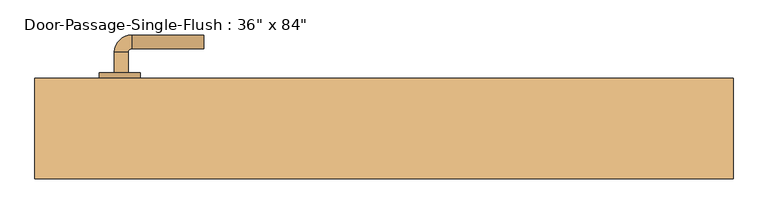
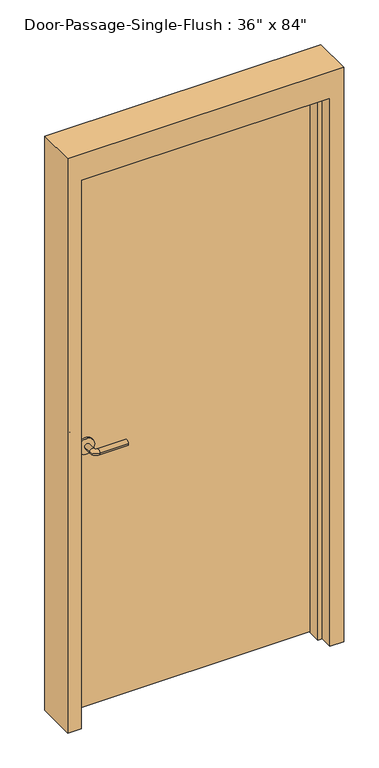
"""IFC4 building model written with IfcOpenShell, lengths in millimetres: door geometry."""

from ifc_helpers import new_model, si_unit, point, frame, frame_2d, origin, origin_with_axes, place, context, project, spatial, polyline, circle_curve, ellipse_curve, trimmed, segment, composite_curve, outline, extrude, faceted_brep, source, transform, mapped, element, save
from ifc_brep_helpers import plane_surface, cylinder_surface, revolved_surface, advanced_brep


def door_a856c21e(model_context):
    return source(origin(), model_context, "Body", "SolidModel", [
        advanced_brep(
        [(-392.190625, 80.9, 1016.0), (-372.190625, 80.9, 1016.0), (-372.190625, 50.9, 1016.0), (-392.190625, 50.9, 1016.0), (-367.190625, 45.9, 1016.0), (-367.190625, 25.9, 1016.0), (-262.190625, 25.9, 1016.0), (-262.190625, 45.9, 1016.0)],
        [
            (0, 1, circle_curve(frame((-382.190625, 80.9, 1016.0), z_axis=(0.0, 1.0, 0.0), x_axis=(1.0, 0.0, 0.0)), 10.0)),
            (1, 0, circle_curve(frame((-382.190625, 80.9, 1016.0), z_axis=(0.0, 1.0, 0.0), x_axis=(1.0, 0.0, 0.0)), 10.0)),
            (1, 2),
            (2, 3, circle_curve(frame((-382.190625, 50.9, 1016.0), z_axis=(0.0, 1.0, 0.0), x_axis=(1.0, 0.0, 0.0)), 10.0)),
            (3, 0),
            (3, 2, circle_curve(frame((-382.190625, 50.9, 1016.0), z_axis=(0.0, 1.0, 0.0), x_axis=(1.0, 0.0, 0.0)), 10.0)),
            (4, 5, circle_curve(frame((-367.190625, 35.9, 1016.0), z_axis=(-1.0, 0.0, 0.0), x_axis=(0.0, 1.0, 0.0)), 10.0)),
            (5, 3, circle_curve(frame((-367.190625, 50.9, 1016.0), z_axis=(0.0, 0.0, -1.0), x_axis=(-1.0, 0.0, 0.0)), 25.0)),
            (2, 4, circle_curve(frame((-367.190625, 50.9, 1016.0), z_axis=(0.0, 0.0, 1.0), x_axis=(-1.0, 0.0, 0.0)), 5.0)),
            (5, 4, circle_curve(frame((-367.190625, 35.9, 1016.0), z_axis=(-1.0, 0.0, 0.0), x_axis=(0.0, 1.0, 0.0)), 10.0)),
            (6, 7, circle_curve(frame((-262.190625, 35.9, 1016.0), z_axis=(1.0, 0.0, 0.0), x_axis=(0.0, 1.0, 0.0)), 10.0)),
            (7, 6, circle_curve(frame((-262.190625, 35.9, 1016.0), z_axis=(1.0, 0.0, 0.0), x_axis=(0.0, 1.0, 0.0)), 10.0)),
            (4, 7),
            (6, 5),
        ],
        [
            plane_surface(frame((-382.190625, 80.9, 1016.0), z_axis=(0.0, 1.0, 0.0), x_axis=(0.0, 0.0, 1.0))),
            cylinder_surface(frame((-382.190625, 80.9, 1016.0), z_axis=(0.0, 1.0, 0.0), x_axis=(1.0, 0.0, 0.0)), 10.0),
            revolved_surface(trimmed(ellipse_curve(frame((-382.190625, 50.9, 1016.0), z_axis=(0.0, -1.0, 0.0), x_axis=(1.0, 0.0, 0.0)), 10.0, 10.0), [point((-392.190625, 50.9, 1016.0))], [point((-372.190625, 50.9, 1016.0))], True, "CARTESIAN"), (-367.190625, 50.9, 1016.0), (0.0, 0.0, -1.0)),
            revolved_surface(trimmed(ellipse_curve(frame((-382.190625, 50.9, 1016.0), z_axis=(0.0, -1.0, 0.0), x_axis=(1.0, 0.0, 0.0)), 10.0, 10.0), [point((-372.190625, 50.9, 1016.0))], [point((-392.190625, 50.9, 1016.0))], True, "CARTESIAN"), (-367.190625, 50.9, 1016.0), (0.0, 0.0, -1.0)),
            plane_surface(frame((-262.190625, 35.9, 1016.0), z_axis=(1.0, 0.0, 0.0), x_axis=(0.0, 0.0, 1.0))),
            cylinder_surface(frame((-367.190625, 35.9, 1016.0), z_axis=(-1.0, 0.0, 0.0), x_axis=(0.0, 1.0, 0.0)), 10.0),
        ],
        [
            (0, [[1, 2]]),
            (1, [[3, 4, 5, -2]]),
            (1, [[-5, 6, -3, -1]]),
            (2, [[7, 8, -4, 9]]),
            (3, [[10, -9, -6, -8]]),
            (4, [[11, 12]]),
            (5, [[13, -11, 14, -7]]),
            (5, [[-14, -12, -13, -10]]),
        ],
    ),
        extrude(outline(composite_curve([segment(trimmed(circle_curve(frame_2d((1016.0, -384.690625)), 30.0), [point((1016.0, -414.690625))], [point((1016.0, -354.690625))], False, "CARTESIAN"), True, "CONTINUOUS"), segment(trimmed(circle_curve(frame_2d((1016.0, -384.690625)), 30.0), [point((1016.0, -354.690625))], [point((1016.0, -414.690625))], False, "CARTESIAN"), True, "CONTINUOUS")], self_intersect=False)), frame((0.0, 80.9, 0.0), z_axis=(0.0, 1.0, 0.0), x_axis=(0.0, 0.0, 1.0)), (0.0, 0.0, 1.0), 8.0),
        advanced_brep(
        [(-392.190625, 141.35, 1016.0), (-372.190625, 141.35, 1016.0), (-392.190625, 171.35, 1016.0), (-372.190625, 171.35, 1016.0), (-367.190625, 176.35, 1016.0), (-367.190625, 196.35, 1016.0), (-262.190625, 196.35, 1016.0), (-262.190625, 176.35, 1016.0)],
        [
            (0, 1, circle_curve(frame((-382.190625, 141.35, 1016.0), z_axis=(0.0, -1.0, 0.0), x_axis=(1.0, 0.0, 0.0)), 10.0)),
            (1, 0, circle_curve(frame((-382.190625, 141.35, 1016.0), z_axis=(0.0, -1.0, 0.0), x_axis=(1.0, 0.0, 0.0)), 10.0)),
            (0, 2),
            (2, 3, circle_curve(frame((-382.190625, 171.35, 1016.0), z_axis=(0.0, -1.0, 0.0), x_axis=(1.0, 0.0, 0.0)), 10.0)),
            (3, 1),
            (3, 2, circle_curve(frame((-382.190625, 171.35, 1016.0), z_axis=(0.0, -1.0, 0.0), x_axis=(1.0, 0.0, 0.0)), 10.0)),
            (4, 3, circle_curve(frame((-367.190625, 171.35, 1016.0), z_axis=(0.0, 0.0, 1.0), x_axis=(-1.0, 0.0, 0.0)), 5.0)),
            (2, 5, circle_curve(frame((-367.190625, 171.35, 1016.0), z_axis=(0.0, 0.0, -1.0), x_axis=(-1.0, 0.0, 0.0)), 25.0)),
            (5, 4, circle_curve(frame((-367.190625, 186.35, 1016.0), z_axis=(-1.0, 0.0, 0.0), x_axis=(0.0, -1.0, 0.0)), 10.0)),
            (4, 5, circle_curve(frame((-367.190625, 186.35, 1016.0), z_axis=(-1.0, 0.0, 0.0), x_axis=(0.0, -1.0, 0.0)), 10.0)),
            (6, 7, circle_curve(frame((-262.190625, 186.35, 1016.0), z_axis=(1.0, 0.0, 0.0), x_axis=(0.0, -1.0, 0.0)), 10.0)),
            (7, 6, circle_curve(frame((-262.190625, 186.35, 1016.0), z_axis=(1.0, 0.0, 0.0), x_axis=(0.0, -1.0, 0.0)), 10.0)),
            (5, 6),
            (7, 4),
        ],
        [
            plane_surface(frame((-382.190625, 141.35, 1016.0), z_axis=(0.0, -1.0, 0.0), x_axis=(0.0, 0.0, 1.0))),
            cylinder_surface(frame((-382.190625, 141.35, 1016.0), z_axis=(0.0, -1.0, 0.0), x_axis=(1.0, 0.0, 0.0)), 10.0),
            revolved_surface(trimmed(ellipse_curve(frame((-382.190625, 171.35, 1016.0), z_axis=(0.0, -1.0, 0.0), x_axis=(1.0, 0.0, 0.0)), 10.0, 10.0), [point((-392.190625, 171.35, 1016.0))], [point((-372.190625, 171.35, 1016.0))], True, "CARTESIAN"), (-367.190625, 171.35, 1016.0), (0.0, 0.0, -1.0)),
            revolved_surface(trimmed(ellipse_curve(frame((-382.190625, 171.35, 1016.0), z_axis=(0.0, -1.0, 0.0), x_axis=(1.0, 0.0, 0.0)), 10.0, 10.0), [point((-372.190625, 171.35, 1016.0))], [point((-392.190625, 171.35, 1016.0))], True, "CARTESIAN"), (-367.190625, 171.35, 1016.0), (0.0, 0.0, -1.0)),
            plane_surface(frame((-262.190625, 186.35, 1016.0), z_axis=(1.0, 0.0, 0.0), x_axis=(0.0, 0.0, 1.0))),
            cylinder_surface(frame((-367.190625, 186.35, 1016.0), z_axis=(-1.0, 0.0, 0.0), x_axis=(0.0, -1.0, 0.0)), 10.0),
        ],
        [
            (0, [[1, 2]]),
            (1, [[-1, 3, 4, 5]]),
            (1, [[-2, -5, 6, -3]]),
            (2, [[7, -4, 8, 9]]),
            (3, [[-8, -6, -7, 10]]),
            (4, [[11, 12]]),
            (5, [[-9, 13, -12, 14]]),
            (5, [[-10, -14, -11, -13]]),
        ],
    ),
        extrude(outline(composite_curve([segment(trimmed(circle_curve(frame_2d((1016.0, -384.690625)), 30.0), [point((1016.0, -414.690625))], [point((1016.0, -354.690625))], False, "CARTESIAN"), True, "CONTINUOUS"), segment(trimmed(circle_curve(frame_2d((1016.0, -384.690625)), 30.0), [point((1016.0, -354.690625))], [point((1016.0, -414.690625))], False, "CARTESIAN"), True, "CONTINUOUS")], self_intersect=False)), frame((0.0, 133.35, 0.0), z_axis=(0.0, 1.0, 0.0), x_axis=(0.0, 0.0, 1.0)), (0.0, 0.0, 1.0), 8.0),
        faceted_brep([(457.2, 84.1375, 0.0), (457.2, 133.35, 0.0), (508.0, 133.35, 0.0), (508.0, -12.7, 0.0), (457.2, -12.7, 0.0), (457.2, 36.5125, 0.0), (441.325, 36.5125, 0.0), (441.325, 84.1375, 0.0), (457.2, 84.1375, 2133.6), (457.2, 133.35, 2133.6), (-457.2, 133.35, 2133.6), (-457.2, 133.35, 0.0), (-508.0, 133.35, 0.0), (-508.0, 133.35, 2235.2), (508.0, 133.35, 2235.2), (508.0, -12.7, 2235.2), (-508.0, -12.7, 2235.2), (-508.0, -12.7, 0.0), (-457.2, -12.7, 0.0), (-457.2, -12.7, 2133.6), (457.2, -12.7, 2133.6), (457.2, 36.5125, 2133.6), (-457.2, 36.5125, 2133.6), (-457.2, 36.5125, 0.0), (-441.325, 36.5125, 0.0), (-441.325, 36.5125, 2117.725), (441.325, 36.5125, 2117.725), (441.325, 84.1375, 2117.725), (-441.325, 84.1375, 2117.725), (-441.325, 84.1375, 0.0), (-457.2, 84.1375, 0.0), (-457.2, 84.1375, 2133.6)], [[[0, 1, 2, 3, 4, 5, 6, 7]], [[1, 0, 8, 9]], [[2, 1, 9, 10, 11, 12, 13, 14]], [[3, 2, 14, 15]], [[4, 3, 15, 16, 17, 18, 19, 20]], [[5, 4, 20, 21]], [[6, 5, 21, 22, 23, 24, 25, 26]], [[7, 6, 26, 27]], [[0, 7, 27, 28, 29, 30, 31, 8]], [[9, 8, 31, 10]], [[20, 19, 22, 21]], [[26, 25, 28, 27]], [[12, 11, 30, 29, 24, 23, 18, 17]], [[11, 10, 31, 30]], [[13, 12, 17, 16]], [[19, 18, 23, 22]], [[25, 24, 29, 28]], [[15, 14, 13, 16]]]),
        extrude(outline(polyline([(457.2, 88.9), (-457.2, 88.9), (-457.2, 133.35), (457.2, 133.35), (457.2, 88.9)])), origin_with_axes(), (0.0, 0.0, 1.0), 2133.6),
    ])


if __name__ == "__main__":
    model = new_model("IFC4")
    model_context = context("Model", 3, world=origin())
    ifc_project = project(units=[si_unit("LENGTHUNIT", "METRE", prefix="MILLI")], contexts=[model_context])
    site = spatial("IfcSite", under=ifc_project)
    building = spatial("IfcBuilding", under=site)
    placement = place(None, origin())
    door_shape = door_a856c21e(model_context)
    element("IfcDoor", 1, ObjectType="Door-Passage-Single-Flush : 36\" x 84\"", at=placement, inside=building, context=model_context, shape_type="MappedRepresentation", body=[
        mapped(door_shape, transform((0.0, 0.0, 0.0), x_axis=(1.0, 0.0, 0.0), y_axis=(0.0, 1.0, 0.0), z_axis=(0.0, 0.0, 1.0))),
    ])
    save(model, "model.ifc")

# Revit data of these elements
# Type "Door-Passage-Single-Flush : 36\" x 84\""
#   Type Mark = "19"
#   Assembly Code = "B2030200"
#   Analytic Construction = "Wooden"
#   Thickness = 0' - 1 3/4"
#   Thermal Resistance (R) = 2.5876 (h·ft²·°F)/BTU
#   Swing Angle [instance default] = 90.00°
#   Strike Height = 3' - 4"
#   Rough Width [instance default] = 3' - 4"
#   Rough Height [instance default] = 7' - 4"
#   MF Opening Height [instance default] = 0' - 4"
#   MF Opening Width [instance default] = 0' - 4"
#   Inset Calculate [instance default] = 0' - 4"
#   Masonry Inset [instance default] = 0' - 1"
#   Height = 7' - 0"
#   Width = 3' - 0"
#   Heat Transfer Coefficient (U) = 0.3865 BTU/(h·ft²·°F)
#   Masonry Frame Depth = 0' - 5 3/4"
#   Masonry Frame [instance default] = yes
#   Function = 1
#   Dry Wall Frame [instance default] = no
#   Panel Material = Wood - Birch
#   Frame Material = Metal - Paint Finish - Grey
#   Door Handle Material = Aluminum
#   Visual Light Transmittance = 0
#   Solar Heat Gain Coefficient = 0
#   Wall Closure = (empty or 0)
# Element 1 (IfcDoor, "Door-Passage-Single-Flush : 36\" x 84\"")
#   Materials on its faces: "Aluminum", "Metal - Paint Finish - Grey", "Wood - Birch"
# Materials
#   "Wood - Birch": class "Wood", colour RGB 166 116 52, transparency 0, Cost = 0
#   "Metal - Paint Finish - Grey": class "Paint", colour RGB 104 104 104, transparency 0, Cost = 0
#   "Aluminum": class "Metal", colour RGB 247 247 247, transparency 0, Description = "Aluminum 6061", Cost = 0
